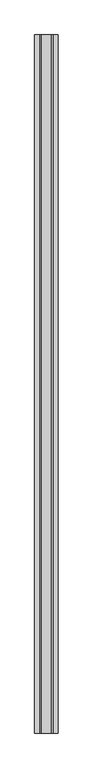
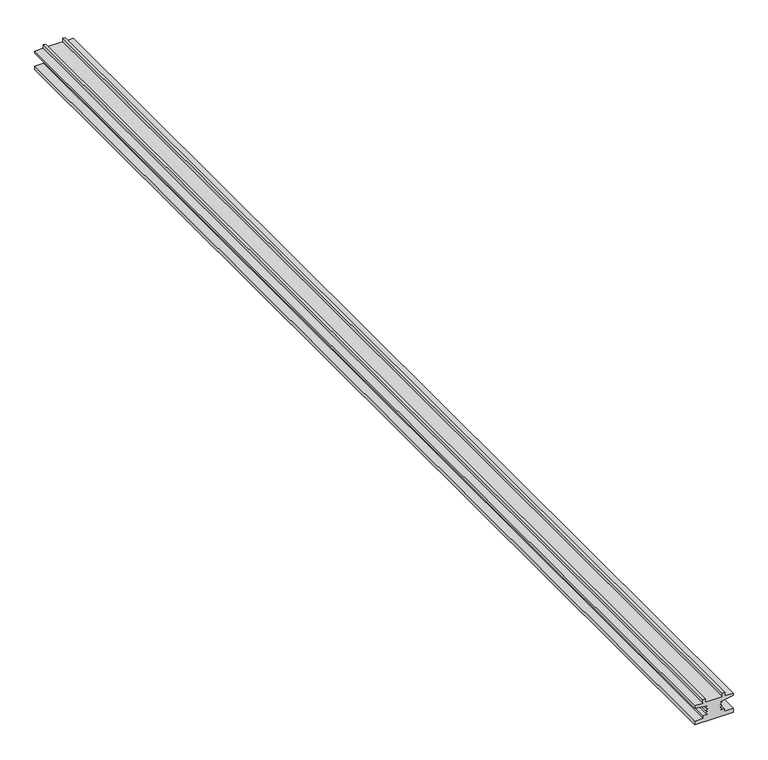
"""IFC4 building model written with IfcOpenShell, lengths in millimetres: proxy geometry, Bison pedestal004 : Bison pedestal004."""

from ifc_helpers import new_model, si_unit, frame, origin, place, context, project, spatial, polyline, outline, extrude, source, transform, mapped, element, save


def generic_models_1fc90002(model_context):
    return source(origin(), model_context, "Body", "SweptSolid", [
        extrude(outline(polyline([(36480.0342739, -2743.0545525), (36486.734375, -2742.9899902), (36486.734375, -2758.4094238), (36491.2120625, -2758.4094238), (36491.2120625, -2766.5004883), (36494.1534688, -2762.9697266), (36496.7296406, -2766.2797852), (36499.4503438, -2762.7492676), (36502.0245625, -2766.1328125), (36504.5577656, -2762.5581055), (36507.1046406, -2765.7746582), (36510.9913594, -2742.9899902), (36515.1456563, -2742.9899902), (36515.1456563, -2757.7331543), (36521.3116719, -2757.7331543), (36521.3116719, -2761.619873), (36515.1456563, -2761.619873), (36515.1456563, -2791.9099121), (36521.3116719, -2791.9099121), (36521.3116719, -2795.7966309), (36515.1456563, -2795.7966309), (36515.1456563, -2810.5397949), (36510.9913594, -2810.5397949), (36507.1046406, -2787.755127), (36504.5577656, -2790.9716797), (36502.0245625, -2787.3969727), (36499.4503438, -2790.7805176), (36496.7296406, -2787.25), (36494.1534688, -2790.5600586), (36491.2120625, -2787.0292969), (36491.2120625, -2795.1203613), (36486.734375, -2795.1203613), (36486.734375, -2810.5397949), (36480.0342739, -2810.4752326), (36480.0342739, -2743.0545525)])), frame((0.0, 998.1570053, 0.0), z_axis=(0.0, 1.0, 0.0), x_axis=(0.0, 0.0, 1.0)), (0.0, 0.0, 1.0), 2000.0),
    ])


if __name__ == "__main__":
    model = new_model("IFC4")
    model_context = context("Model", 3, world=origin())
    ifc_project = project(units=[si_unit("LENGTHUNIT", "METRE", prefix="MILLI")], contexts=[model_context])
    site = spatial("IfcSite", under=ifc_project)
    building = spatial("IfcBuilding", under=site)
    placement = place(None, origin())
    generic_models_shape = generic_models_1fc90002(model_context)
    element("IfcBuildingElementProxy", 1, Name="Bison pedestal004 : Bison pedestal004", ObjectType="Bison pedestal004 : Bison pedestal004", at=placement, inside=building, context=model_context, shape_type="MappedRepresentation", body=[
        mapped(generic_models_shape, transform((0.0, 0.0, 0.0), x_axis=(1.0, 0.0, 0.0), y_axis=(0.0, 1.0, 0.0), z_axis=(0.0, 0.0, 1.0))),
    ])
    save(model, "model.ifc")

# Revit data of these elements
# Type "Bison pedestal004 : Bison pedestal004"
#   NameOverride = "Bison pedestal004"
# Element 1 (IfcBuildingElementProxy, "Bison pedestal004 : Bison pedestal004")
#   Materials on its faces: "BUZON PEDESTAL"
# Materials
#   "BUZON PEDESTAL": class "Unassigned", colour RGB 66 66 66, transparency 0
